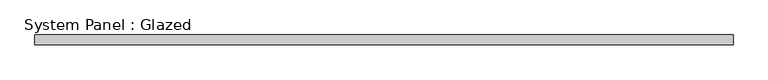
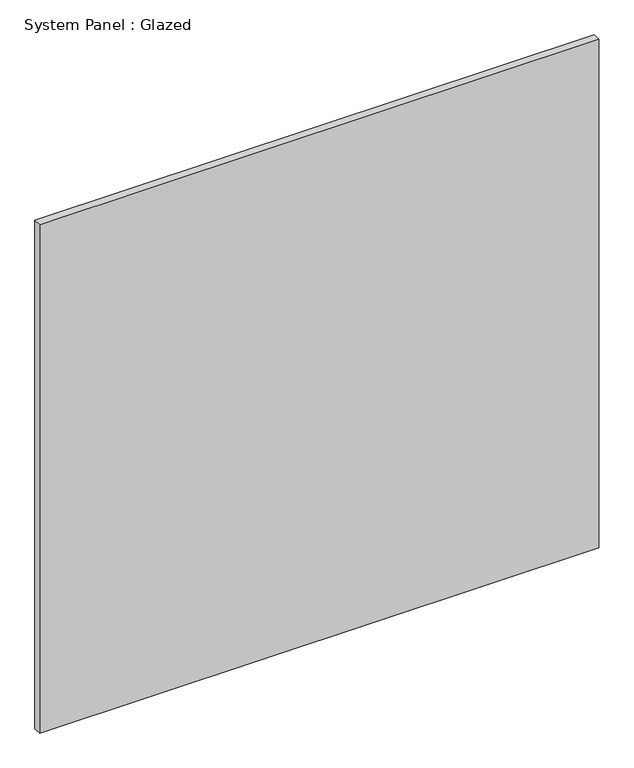
"""IFC4 building model written with IfcOpenShell, lengths in millimetres: plate geometry, System Panel : Glazed."""

from ifc_helpers import new_model, si_unit, origin, origin_with_axes, place, context, project, spatial, polyline, outline, extrude, source, transform, mapped, element, save


def system_panel_glazed_6f098d11(model_context):
    return source(origin(), model_context, "Body", "SweptSolid", [
        extrude(outline(polyline([(877.5000002, 24.5), (-877.5000002, 24.5), (-877.5000002, 49.5), (877.5000002, 49.5), (877.5000002, 24.5)])), origin_with_axes(), (0.0, 0.0, 1.0), 1686.2355347),
    ])


if __name__ == "__main__":
    model = new_model("IFC4")
    model_context = context("Model", 3, world=origin())
    ifc_project = project(units=[si_unit("LENGTHUNIT", "METRE", prefix="MILLI")], contexts=[model_context])
    site = spatial("IfcSite", under=ifc_project)
    building = spatial("IfcBuilding", under=site)
    placement = place(None, origin())
    system_panel_glazed_shape = system_panel_glazed_6f098d11(model_context)
    element("IfcPlate", 1, ObjectType="System Panel : Glazed", at=placement, inside=building, context=model_context, shape_type="MappedRepresentation", body=[
        mapped(system_panel_glazed_shape, transform((0.0, 0.0, 0.0), x_axis=(1.0, 0.0, 0.0), y_axis=(0.0, 1.0, 0.0), z_axis=(0.0, 0.0, 1.0))),
    ])
    save(model, "model.ifc")

# Revit data of these elements
# Element 1 (IfcPlate, "System Panel : Glazed")
#   Materials on its faces: "Glass"
# Materials
#   "Glass": class "Glass", colour RGB 218 227 224, transparency 0.85, Description = "Soda Lime Glass", Cost = 0
